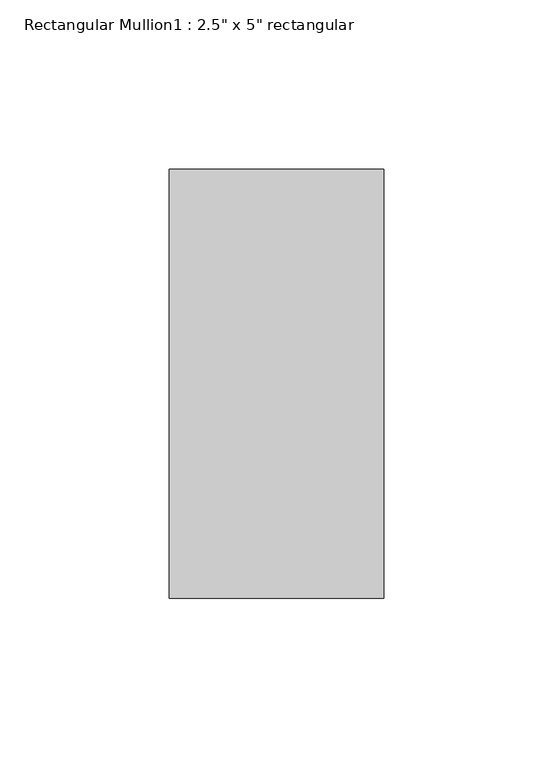
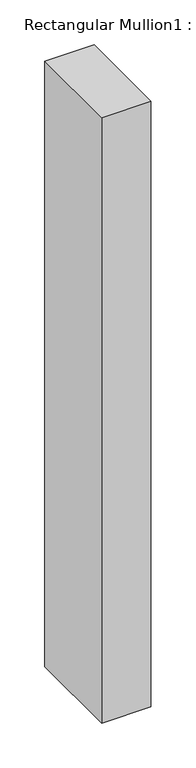
"""IFC4 building model written with IfcOpenShell, lengths in millimetres: member geometry."""

import ifcopenshell
import ifcopenshell.guid

model = None  # the IFC model being written
_history = None  # IfcOwnerHistory: only IFC2X3 demands one
_inside = {}  # id of a spatial element -> (the spatial element, [elements in it])
_under = {}  # id of a project, library or spatial element -> (it, [spatial elements below it])
_declared = {}  # id of a project -> (the project, [libraries it declares])
_typed = {}  # id of a type object -> (the type object, [elements of that type])
_made_of = {}  # id of a material, layer set ... -> (it, [elements and type objects made of it])


def new_model(schema):
    """Start an empty IFC model of exactly this schema.

    Asked for "IFC4X3", IfcOpenShell would pick the latest addendum, in which some entities
    have other attributes; the version numbers below select the first issue.
    IFC2X3 requires an IfcOwnerHistory on every rooted entity: one is made here for all.
    """
    global model, _history
    if schema == "IFC4X3":
        model = ifcopenshell.file(schema_version=(4, 3, 0, 0))
    else:
        model = ifcopenshell.file(schema=schema)
    _inside.clear()
    _under.clear()
    _declared.clear()
    _typed.clear()
    _made_of.clear()
    _history = None
    if model.schema == "IFC2X3":
        org = make("IfcOrganization", Name="unknown")
        user = make(
            "IfcPersonAndOrganization",
            ThePerson=make("IfcPerson", FamilyName="unknown"),
            TheOrganization=org,
        )
        app = make(
            "IfcApplication",
            ApplicationDeveloper=org,
            Version="unknown",
            ApplicationFullName="unknown",
            ApplicationIdentifier="unknown",
        )
        _history = make(
            "IfcOwnerHistory",
            OwningUser=user,
            OwningApplication=app,
            ChangeAction="ADDED",
            CreationDate=0,
        )
    return model


def make(cls, **values):
    """One entity of the class cls with the attributes given. An attribute that is None is left unset."""
    return model.create_entity(
        cls, **{name: value for name, value in values.items() if value is not None}
    )


def rooted(cls, **values):
    """An entity with a GlobalId (a new one), such as an element, a storey or a relation."""
    return make(cls, GlobalId=ifcopenshell.guid.new(), OwnerHistory=_history, **values)


def si_unit(unit_type, name, prefix=None):
    """IfcSIUnit, for example si_unit("LENGTHUNIT", "METRE", prefix="MILLI")."""
    return make("IfcSIUnit", UnitType=unit_type, Prefix=prefix, Name=name)


def assignment(units):
    """IfcUnitAssignment: the units of a project."""
    return None if units is None else make("IfcUnitAssignment", Units=units)


def point(xyz):
    """IfcCartesianPoint."""
    return None if xyz is None else make("IfcCartesianPoint", Coordinates=xyz)


def direction(xyz):
    """IfcDirection."""
    return None if xyz is None else make("IfcDirection", DirectionRatios=xyz)


def frame(location, z_axis=None, x_axis=None):
    """IfcAxis2Placement3D, a coordinate frame: its origin and axes. An axis left out is left unset."""
    return make(
        "IfcAxis2Placement3D",
        Location=point(location),
        Axis=direction(z_axis),
        RefDirection=direction(x_axis),
    )


def origin():
    """The frame at (0, 0, 0) with its axes left unset."""
    return frame((0.0, 0.0, 0.0))


def place(relative_to, where):
    """IfcLocalPlacement: puts the frame where relative to a parent placement (None: the world)."""
    return make(
        "IfcLocalPlacement", PlacementRelTo=relative_to, RelativePlacement=where
    )


def context(
    kind, dimensions, precision=None, world=None, true_north=None, identifier=None
):
    """IfcGeometricRepresentationContext, for example the 3D "Model" context."""
    return make(
        "IfcGeometricRepresentationContext",
        ContextIdentifier=identifier,
        ContextType=kind,
        CoordinateSpaceDimension=dimensions,
        Precision=precision,
        WorldCoordinateSystem=world,
        TrueNorth=true_north,
    )


def project(units=None, contexts=None):
    """IfcProject with its units and contexts."""
    return rooted(
        "IfcProject",
        Name="project",
        RepresentationContexts=contexts,
        UnitsInContext=assignment(units),
    )


def spatial(cls, under=None, at=None, **own):
    """A site, building, storey or space (cls), placed at a placement, below another one or the project."""
    s = rooted(cls, ObjectPlacement=at, **own)
    if under is not None:
        _under.setdefault(under.id(), (under, []))[1].append(s)
    return s


def polyline(points):
    """IfcPolyline through the points."""
    return make("IfcPolyline", Points=[point(p) for p in points])


def outline(outer, holes=None, kind="AREA"):
    """IfcArbitraryClosedProfileDef: a profile drawn as a closed curve; with holes, ...WithVoids."""
    if holes is None:
        return make("IfcArbitraryClosedProfileDef", ProfileType=kind, OuterCurve=outer)
    return make(
        "IfcArbitraryProfileDefWithVoids",
        ProfileType=kind,
        OuterCurve=outer,
        InnerCurves=holes,
    )


def extrude(swept, where, along, depth):
    """IfcExtrudedAreaSolid: the profile swept, set in the frame where, extruded along a direction by depth."""
    return make(
        "IfcExtrudedAreaSolid",
        SweptArea=swept,
        Position=where,
        ExtrudedDirection=direction(along),
        Depth=depth,
    )


def shape(context_of_items, identifier, shape_type, items):
    """IfcShapeRepresentation: the items that make up one representation, for example the "Body"."""
    return make(
        "IfcShapeRepresentation",
        ContextOfItems=context_of_items,
        RepresentationIdentifier=identifier,
        RepresentationType=shape_type,
        Items=items,
    )


def source(mapping_origin, context_of_items, identifier, shape_type, items):
    """IfcRepresentationMap: a shape defined once, which mapped items show again and again."""
    return make(
        "IfcRepresentationMap",
        MappingOrigin=mapping_origin,
        MappedRepresentation=shape(context_of_items, identifier, shape_type, items),
    )


def transform(
    local_origin,
    x_axis=None,
    y_axis=None,
    z_axis=None,
    scale=None,
    scale2=None,
    scale3=None,
    uniform=True,
):
    """IfcCartesianTransformationOperator3D, or its non-uniform kind. x_axis, y_axis, z_axis: its Axis1, 2, 3."""
    if uniform:
        return make(
            "IfcCartesianTransformationOperator3D",
            Axis1=direction(x_axis),
            Axis2=direction(y_axis),
            LocalOrigin=point(local_origin),
            Scale=scale,
            Axis3=direction(z_axis),
        )
    return make(
        "IfcCartesianTransformationOperator3DnonUniform",
        Axis1=direction(x_axis),
        Axis2=direction(y_axis),
        LocalOrigin=point(local_origin),
        Scale=scale,
        Axis3=direction(z_axis),
        Scale2=scale2,
        Scale3=scale3,
    )


def mapped(mapping_source, mapping_target):
    """IfcMappedItem: shows the shape of a source again, moved by a transform."""
    return make(
        "IfcMappedItem", MappingSource=mapping_source, MappingTarget=mapping_target
    )


def made_of(thing, what):
    """Note that an element or type object is made of a material, layer set ...; save() writes the relation."""
    if what is not None:
        _made_of.setdefault(what.id(), (what, []))[1].append(thing)
    return thing


def element(
    cls,
    number,
    at=None,
    inside=None,
    cuts=None,
    type_object=None,
    material=None,
    context=None,
    identifier="Body",
    shape_type=None,
    held_by="IfcProductDefinitionShape",
    body=None,
    shapes=None,
    **own,
):
    """One element of the class cls, such as IfcWall. Its Tag is "e" and its number.

    at: its placement. inside: the storey or other place that contains it. cuts: it is an
    opening in that element (IfcRelVoidsElement). A single representation is given by context,
    identifier, shape_type and body (its items); several are given by shapes. held_by: the class
    of the entity that holds the representations. save() writes the other relations.
    """
    e = rooted(cls, Tag="e%d" % number, ObjectPlacement=at, **own)
    if body is not None:
        shapes = [shape(context, identifier, shape_type, body)]
    if shapes is not None:
        e.Representation = make(held_by, Representations=shapes)
    if inside is not None:
        _inside.setdefault(inside.id(), (inside, []))[1].append(e)
    if cuts is not None:
        rooted(
            "IfcRelVoidsElement", RelatingBuildingElement=cuts, RelatedOpeningElement=e
        )
    if type_object is not None:
        _typed.setdefault(type_object.id(), (type_object, []))[1].append(e)
    return made_of(e, material)


def aggregate(whole, parts):
    """IfcRelAggregates: a whole, such as a stair, and the parts it consists of."""
    return rooted("IfcRelAggregates", RelatingObject=whole, RelatedObjects=parts)


def save(model, path):
    """Write the relations noted so far, then the file.

    IfcRelAggregates (storeys below a building ...), IfcRelContainedInSpatialStructure (elements
    in a storey), IfcRelDefinesByType, IfcRelAssociatesMaterial and IfcRelDeclares: one each for
    every whole, place, type object, material and project.
    """
    for whole, parts in _under.values():
        aggregate(whole, parts)
    for where, things in _inside.values():
        rooted(
            "IfcRelContainedInSpatialStructure",
            RelatedElements=things,
            RelatingStructure=where,
        )
    for kind, things in _typed.values():
        rooted("IfcRelDefinesByType", RelatedObjects=things, RelatingType=kind)
    for what, things in _made_of.values():
        rooted("IfcRelAssociatesMaterial", RelatedObjects=things, RelatingMaterial=what)
    for by, libraries in _declared.values():
        rooted("IfcRelDeclares", RelatingContext=by, RelatedDefinitions=libraries)
    model.write(path)


def member_74aba05d(model_context):
    return source(origin(), model_context, "Body", "SweptSolid", [
        extrude(outline(polyline([(31.75, 63.5), (31.75, -63.5), (-31.75, -63.5), (-31.75, 63.5), (31.75, 63.5)])), frame((0.0, 0.0, -825.5), z_axis=(0.0, 0.0, 1.0), x_axis=(1.0, 0.0, 0.0)), (0.0, 0.0, 1.0), 825.5),
    ])


if __name__ == "__main__":
    model = new_model("IFC4")
    model_context = context("Model", 3, world=origin())
    ifc_project = project(units=[si_unit("LENGTHUNIT", "METRE", prefix="MILLI")], contexts=[model_context])
    site = spatial("IfcSite", under=ifc_project)
    building = spatial("IfcBuilding", under=site)
    placement = place(None, origin())
    member_shape = member_74aba05d(model_context)
    element("IfcMember", 1, ObjectType="Rectangular Mullion1 : 2.5\" x 5\" rectangular", at=placement, inside=building, context=model_context, shape_type="MappedRepresentation", body=[
        mapped(member_shape, transform((0.0, 0.0, 0.0), x_axis=(1.0, 0.0, 0.0), y_axis=(0.0, 1.0, 0.0), z_axis=(0.0, 0.0, 1.0))),
    ])
    save(model, "model.ifc")

# Revit data of these elements
# Type "Rectangular Mullion1 : 2.5\" x 5\" rectangular"
#   built-in parameter 1007304 = 0.416667 (stored number, unit not read)
#   built-in parameter 1007301 = 0.104167 (stored number, unit not read)
#   built-in parameter 1007300 = 0.104167 (stored number, unit not read)
# Element 1 (IfcMember, "Rectangular Mullion1 : 2.5\" x 5\" rectangular")
#   Materials on its faces: "support-frame"
# Materials
#   "support-frame": class "Unassigned", colour RGB 233 233 233, transparency 0, Cost = 0
